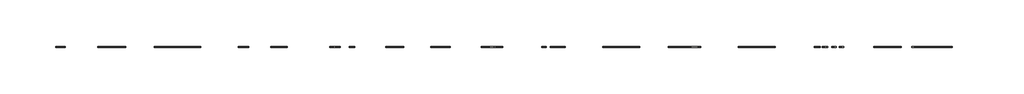
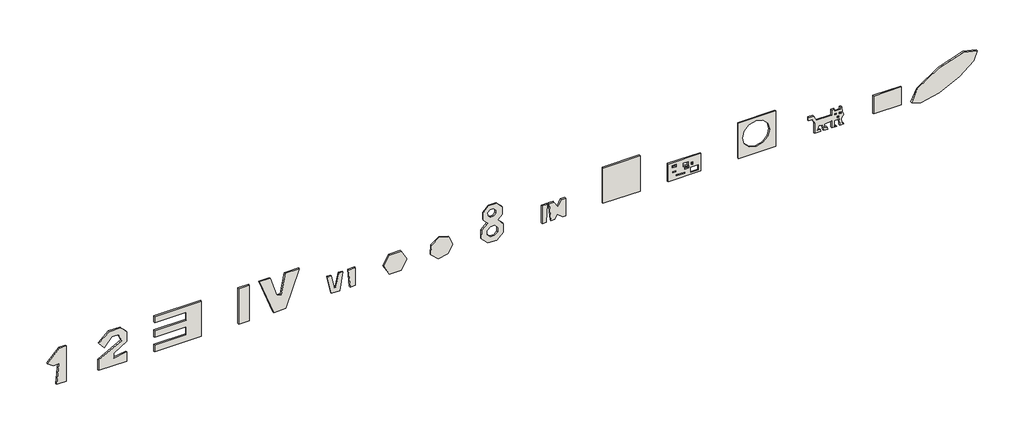
# One storey: 15 walls.
"""IFC4 building model written with IfcOpenShell, lengths in millimetres."""

from ifc_helpers import new_model, si_unit, point, frame, origin, origin_with_axes, place, context, project, spatial, polyline, ellipse_curve, trimmed, outline, extrude, element, save
from ifc_brep_helpers import plane_surface, extruded_surface, advanced_brep

model = new_model("IFC4")

# Units and contexts
model_context = context("Model", 3, world=origin())
ifc_project = project(units=[si_unit("LENGTHUNIT", "METRE", prefix="MILLI")], contexts=[model_context])

# Site, building, storey
site = spatial("IfcSite", under=ifc_project)
building = spatial("IfcBuilding", under=site)
storey = spatial("IfcBuildingStorey", under=building, Name="1 етаж", Elevation=0.0)

# Walls
placement = place(None, origin())
element("IfcWall", 1, ObjectType="Cav - 102 75i 100 p - Lwt", at=placement, inside=storey, context=model_context, shape_type="SweptSolid", body=[
    extrude(outline(polyline([(0.0, -98630.5096965), (8000.0, -98630.5096965), (8000.0, -100030.5096965), (5400.0, -102630.5096965), (4539.6353455, -101401.7816301), (4539.6353455, -100201.7816301), (0.0, -100630.5096965), (0.0, -98630.5096965)])), frame((0.0, 42970.9466245, 0.0), z_axis=(0.0, 1.0, 0.0), x_axis=(0.0, 0.0, 1.0)), (0.0, 0.0, 1.0), 290.0),
])
element("IfcWall", 2, ObjectType="Cav - 102 75i 100 p - Lwt", at=placement, inside=storey, context=model_context, shape_type="SweptSolid", body=[
    extrude(outline(polyline([(0.0, -91630.5096965), (0.0, -85630.5096965), (2094.5145842, -85630.5096965), (1651.266428, -88429.0684139), (2751.266428, -88429.0684139), (4500.0, -85630.5096965), (6700.0, -85630.5096965), (8000.0, -86930.5096965), (8000.0, -89366.1778706), (6130.4395076, -91594.233304), (4690.3678843, -90385.869736), (6660.3947683, -88846.7160477), (6660.3947683, -87446.7160477), (5029.0407516, -86686.0031765), (2400.0, -91630.5096965), (0.0, -91630.5096965)])), frame((0.0, 42970.9466245, 0.0), z_axis=(0.0, 1.0, 0.0), x_axis=(0.0, 0.0, 1.0)), (0.0, 0.0, 1.0), 290.0),
])
element("IfcWall", 3, ObjectType="Cav - 102 75i 100 p - Lwt", at=placement, inside=storey, context=model_context, shape_type="SweptSolid", body=[
    extrude(outline(polyline([(6600.0, -79630.5096965), (6600.0, -72830.5096965), (4800.0, -72830.5096965), (4800.0, -79630.5096965), (3300.0, -79630.5096965), (3300.0, -72830.5096965), (1500.0, -72830.5096965), (1500.0, -79630.5096965), (0.0, -79630.5096965), (0.0, -69630.5096965), (8000.0, -69630.5096965), (8000.0, -79630.5096965), (6600.0, -79630.5096965)])), frame((0.0, 42970.9466245, 0.0), z_axis=(0.0, 1.0, 0.0), x_axis=(0.0, 0.0, 1.0)), (0.0, 0.0, 1.0), 290.0),
])
element("IfcWall", 4, ObjectType="Cav - 102 75i 100 p - Lwt", at=placement, inside=storey, context=model_context, shape_type="SweptSolid", body=[
    extrude(outline(polyline([(-59330.5096965, 42970.9466245), (-61630.5096965, 42970.9466245), (-61630.5096965, 43260.9466245), (-59330.5096965, 43260.9466245), (-59330.5096965, 42970.9466245)])), origin_with_axes(), (0.0, 0.0, 1.0), 8000.0),
    extrude(outline(polyline([(8000.0, -51722.1990601), (3451.4918474, -52524.2237694), (3625.140025, -53509.0315224), (8000.0, -54930.5096965), (8000.0, -57230.5096965), (0.0, -54159.5974163), (0.0, -51542.2715707), (8000.0, -48630.5096965), (8000.0, -51722.1990601)])), frame((0.0, 42970.9466245, 0.0), z_axis=(0.0, 1.0, 0.0), x_axis=(0.0, 0.0, 1.0)), (0.0, 0.0, 1.0), 290.0),
])
element("IfcWall", 5, ObjectType="Cav - 102 75i 100 p - Lwt", at=placement, inside=storey, context=model_context, shape_type="SweptSolid", body=[
    extrude(outline(polyline([(4000.0, -36630.5096965), (4000.0, -38130.5096965), (0.0, -37780.5550424), (0.0, -36630.5096965), (4000.0, -36630.5096965)])), frame((0.0, 42970.9466245, 0.0), z_axis=(0.0, 1.0, 0.0), x_axis=(0.0, 0.0, 1.0)), (0.0, 0.0, 1.0), 290.0),
    extrude(outline(polyline([(0.0, -39964.0474578), (4000.0, -39330.5096965), (4000.0, -40183.0395516), (1065.5571978, -40806.7746241), (1065.5571978, -41206.7746241), (4000.0, -41830.5096965), (4000.0, -42630.5096965), (0.0, -41780.2834499), (0.0, -39964.0474578)])), frame((0.0, 42970.9466245, 0.0), z_axis=(0.0, 1.0, 0.0), x_axis=(0.0, 0.0, 1.0)), (0.0, 0.0, 1.0), 290.0),
])
element("IfcWall", 6, ObjectType="Cav - 102 75i 100 p - Lwt", at=placement, inside=storey, context=model_context, shape_type="SweptSolid", body=[
    extrude(outline(polyline([(21.877764, -26870.6721957), (2169.9022222, -25630.5096965), (4317.9266805, -26870.6721957), (4317.9266805, -29350.9971941), (2169.9022222, -30591.1596933), (21.877764, -29350.9971941), (21.877764, -26870.6721957)])), frame((0.0, 42970.9466245, 0.0), z_axis=(0.0, 1.0, 0.0), x_axis=(0.0, 0.0, 1.0)), (0.0, 0.0, 1.0), 290.0),
])
element("IfcWall", 7, ObjectType="Cav - 102 75i 100 p - Lwt", at=placement, inside=storey, context=model_context, shape_type="SweptSolid", body=[
    extrude(outline(polyline([(2063.3424206, -15809.1102472), (4000.0, -16630.5096965), (4565.2903012, -18656.7837428), (3333.5381977, -20362.1067006), (1232.2781465, -20462.3356006), (-156.1981759, -18881.9960367), (213.660221, -16811.1159336), (2063.3424206, -15809.1102472)])), frame((0.0, 42970.9466245, 0.0), z_axis=(0.0, 1.0, 0.0), x_axis=(0.0, 0.0, 1.0)), (0.0, 0.0, 1.0), 290.0),
])
element("IfcWall", 8, ObjectType="Cav - 102 75i 100 p - Lwt", at=placement, inside=storey, context=model_context, shape_type="SweptSolid", body=[
    extrude(outline(polyline([(6805.7289018, -5192.4839493), (8000.0, -6366.0908889), (8014.6117667, -8040.4335066), (6841.004827, -9234.7046048), (5166.6622094, -9249.3163715), (4214.4462038, -8313.576309), (3005.9972917, -9587.015755), (1085.0591362, -9637.3172909), (-308.8178169, -8314.5774521), (-359.1193527, -6393.6392966), (963.6204861, -4999.7623435), (2884.5586416, -4949.4608076), (4178.1921217, -6177.0731426), (5131.3862841, -5207.0957159), (6805.7289018, -5192.4839493)]), holes=[polyline([(5866.8485377, -6578.1456906), (5358.9896583, -7043.5126137), (5328.943308, -7731.6871783), (5794.3102311, -8239.5460576), (6482.4847957, -8269.592408), (6990.343675, -7804.2254848), (7020.3900254, -7116.0509203), (6555.0231022, -6608.1920409), (5866.8485377, -6578.1456906)]), polyline([(3115.8715667, -6771.7493574), (2438.7263942, -6151.2601266), (1521.1603081, -6191.321927), (900.6710773, -6868.4670995), (940.7328778, -7786.0331856), (1617.8780502, -8406.5224164), (2535.4441363, -8366.4606159), (3155.9333672, -7689.3154435), (3115.8715667, -6771.7493574)])]), frame((0.0, 42970.9466245, 0.0), z_axis=(0.0, 1.0, 0.0), x_axis=(0.0, 0.0, 1.0)), (0.0, 0.0, 1.0), 290.0),
])
element("IfcWall", 9, ObjectType="Cav - 102 75i 100 p - Lwt", at=placement, inside=storey, context=model_context, shape_type="SweptSolid", body=[
    extrude(outline(polyline([(0.0, 3369.4903035), (0.0, 4259.8591863), (4000.0, 4469.4903035), (4000.0, 3369.4903035), (0.0, 3369.4903035)])), frame((0.0, 42970.9466245, 0.0), z_axis=(0.0, 1.0, 0.0), x_axis=(0.0, 0.0, 1.0)), (0.0, 0.0, 1.0), 290.0),
    extrude(outline(polyline([(4000.0, 8369.4903035), (4000.0, 7408.7244661), (2643.1230461, 6717.3611262), (4000.0, 5869.4903035), (4000.0, 4869.4903035), (0.0, 5219.4449576), (0.0, 6089.0365293), (989.5288889, 6593.2266812), (0.0, 7772.5012895), (0.0, 8369.4903035), (4000.0, 8369.4903035)])), frame((0.0, 42970.9466245, 0.0), z_axis=(0.0, 1.0, 0.0), x_axis=(0.0, 0.0, 1.0)), (0.0, 0.0, 1.0), 290.0),
])
element("IfcWall", 10, ObjectType="Cav - 102 75i 100 p - Lwt", at=placement, inside=storey, context=model_context, shape_type="SweptSolid", body=[
    extrude(outline(polyline([(24369.4903035, 42970.9466245), (16369.4903035, 42970.9466245), (16369.4903035, 43260.9466245), (24369.4903035, 43260.9466245), (24369.4903035, 42970.9466245)])), origin_with_axes(), (0.0, 0.0, 1.0), 8000.0),
])
element("IfcWall", 11, ObjectType="Cav - 102 75i 100 p - Lwt", at=placement, inside=storey, context=model_context, shape_type="SweptSolid", body=[
    extrude(outline(polyline([(0.0, 30369.4903035), (0.0, 37369.4903035), (4000.0, 37369.4903035), (4000.0, 30369.4903035), (0.0, 30369.4903035)]), holes=[polyline([(3368.16, 32060.8162862), (2868.16, 32060.8162862), (2868.16, 31260.8162862), (3368.16, 31260.8162862), (3368.16, 32060.8162862)]), polyline([(3099.8933333, 34632.1407307), (2299.8933333, 34632.1407307), (2299.8933333, 33532.1407307), (3099.8933333, 33532.1407307), (3099.8933333, 34632.1407307)]), polyline([(962.7022222, 33860.8162862), (762.7022222, 33860.8162862), (762.7022222, 32060.8162862), (962.7022222, 32060.8162862), (962.7022222, 33860.8162862)]), polyline([(1651.2533333, 36822.2207307), (451.2533333, 36822.2207307), (451.2533333, 35222.2207307), (1651.2533333, 35222.2207307), (1651.2533333, 36822.2207307)]), polyline([(2688.5511111, 35324.6207307), (2688.5511111, 35624.6207307), (2188.5511111, 35624.6207307), (2188.5511111, 35324.6207307), (2688.5511111, 35324.6207307)]), polyline([(2125.1911111, 33860.8162862), (2125.1911111, 34703.5718418), (1651.2533333, 34703.5718418), (1651.2533333, 33860.8162862), (2125.1911111, 33860.8162862)]), polyline([(1731.7333333, 31331.4829529), (1931.7333333, 31331.4829529), (1931.7333333, 31931.4829529), (1731.7333333, 31931.4829529), (1731.7333333, 31331.4829529)])]), frame((0.0, 42970.9466245, 0.0), z_axis=(0.0, 1.0, 0.0), x_axis=(0.0, 0.0, 1.0)), (0.0, 0.0, 1.0), 290.0),
])
element("IfcWall", 12, ObjectType="Cav - 102 75i 100 p - Lwt", at=placement, inside=storey, context=model_context, shape_type="SweptSolid", body=[
    extrude(outline(polyline([(0.0, 45369.4903035), (0.0, 53369.4903035), (8000.0, 53369.4903035), (8000.0, 45369.4903035), (0.0, 45369.4903035)]), holes=[polyline([(4318.9511111, 52086.5671726), (2869.5644585, 51698.2051895), (1808.539789, 50637.18052), (1420.177806, 49187.7938674), (1808.539789, 47738.4072148), (2869.5644585, 46677.3825453), (4318.9511111, 46289.0205623), (5768.3377637, 46677.3825453), (6829.3624332, 47738.4072148), (7217.7244163, 49187.7938674), (6829.3624332, 50637.18052), (5768.3377637, 51698.2051895), (4318.9511111, 52086.5671726)])]), frame((0.0, 42970.9466245, 0.0), z_axis=(0.0, 1.0, 0.0), x_axis=(0.0, 0.0, 1.0)), (0.0, 0.0, 1.0), 290.0),
])
element("IfcWall", 13, ObjectType="Cav - 102 75i 100 p - Lwt", at=placement, inside=storey, context=model_context, shape_type="SweptSolid", body=[
    extrude(outline(polyline([(3300.0, 60369.4903035), (3300.0, 61169.4903035), (2337.9183221, 61702.7808857), (0.0, 61702.7808857), (0.0, 62998.7101733), (482.9629131, 62869.3006507), (535.2563588, 62271.5838319), (1458.9577164, 62607.7836314), (1337.403992, 63297.1490585), (0.0, 63655.5053781), (0.0, 64502.7808857), (482.9629131, 64373.3713632), (688.1749991, 63809.5557907), (1385.5112878, 63748.5467708), (1527.3254711, 65369.4903035), (0.0, 65369.4903035), (0.0, 66420.201364), (318.1483442, 65869.1522675), (1418.1483442, 65869.1522675), (1418.1483442, 66969.1522675), (0.0, 67093.2241708), (0.0, 67969.4903035), (494.9747468, 67474.5155566), (1418.1483442, 67393.7483324), (2155.3851841, 67909.9671251), (2816.8665248, 67587.3411185), (4000.0, 67483.830352), (4000.0, 67169.4903035), (3500.0, 67169.4903035), (3500.0, 65969.4903035), (4000.0, 65969.4903035), (4000.0, 65369.4903035), (2800.0, 65369.4903035), (2800.0, 62069.4903035), (4000.0, 61484.2111972), (4000.0, 60369.4903035), (3300.0, 60369.4903035)]), holes=[polyline([(2950.3577045, 66363.1028194), (2650.3577045, 66363.1028194), (2650.3577045, 66063.1028194), (2950.3577045, 66063.1028194), (2950.3577045, 66363.1028194)]), polyline([(2950.3577045, 67384.3679411), (2550.3577045, 67384.3679411), (2550.3577045, 66984.3679411), (2950.3577045, 66984.3679411), (2950.3577045, 67384.3679411)]), polyline([(2164.8579691, 66909.1890889), (1864.8579691, 66909.1890889), (1864.8579691, 66509.1890889), (2164.8579691, 66509.1890889), (2164.8579691, 66909.1890889)])]), frame((0.0, 42970.9466245, 0.0), z_axis=(0.0, 1.0, 0.0), x_axis=(0.0, 0.0, 1.0)), (0.0, 0.0, 1.0), 290.0),
])
element("IfcWall", 14, ObjectType="Cav - 102 75i 100 p - Lwt", at=placement, inside=storey, context=model_context, shape_type="SweptSolid", body=[
    extrude(outline(polyline([(80296.0426464, 42970.9466245), (74369.4903035, 42970.9466245), (74369.4903035, 43260.9466245), (80296.0426464, 43260.9466245), (80296.0426464, 42970.9466245)])), origin_with_axes(), (0.0, 0.0, 1.0), 4000.0),
])
element("IfcWall", 15, ObjectType="Cav - 102 75i 100 p - Lwt", at=placement, inside=storey, context=model_context, shape_type="AdvancedBrep", body=[
    advanced_brep(
    [(96500.2659618, 42970.9466245, 6549.4282783), (82479.0788395, 42970.9466245, -289.1616116), (96500.2659618, 43260.9466245, 6549.4282783), (82479.0788395, 43260.9466245, -289.1616116)],
    [
        (0, 1, ellipse_curve(frame((89489.6724007, 42970.9466245, 3130.1333333), z_axis=(0.0, -1.0000000000000002, 0.0), x_axis=(-0.8987940462991659, 0.0, -0.4383711467890798)), 7800.0, 2600.0)),
        (1, 0, ellipse_curve(frame((89489.6724007, 42970.9466245, 3130.1333333), z_axis=(0.0, -1.0000000000000002, 0.0), x_axis=(-0.8987940462991659, 0.0, -0.4383711467890798)), 7800.0, 2600.0)),
        (2, 3, ellipse_curve(frame((89489.6724007, 43260.9466245, 3130.1333333), z_axis=(0.0, 1.0000000000000002, 0.0), x_axis=(-0.8987940462991659, 0.0, -0.4383711467890798)), 7800.0, 2600.0)),
        (3, 2, ellipse_curve(frame((89489.6724007, 43260.9466245, 3130.1333333), z_axis=(0.0, 1.0000000000000002, 0.0), x_axis=(-0.8987940462991659, 0.0, -0.4383711467890798)), 7800.0, 2600.0)),
        (0, 2),
        (3, 1),
    ],
    [
        plane_surface(frame((82479.0788395, 42970.9466245, -289.1616116), z_axis=(0.0, -1.0000000000000002, 0.0), x_axis=(0.4383711467890798, 0.0, -0.8987940462991659))),
        plane_surface(frame((82479.0788395, 43260.9466245, -289.1616116), z_axis=(0.0, 1.0000000000000002, 0.0), x_axis=(-0.4383711467890798, 0.0, 0.8987940462991659))),
        extruded_surface(trimmed(ellipse_curve(frame((89489.6724007, 43550.9466245, 3130.1333333), z_axis=(0.0, -1.0000000000000002, 0.0), x_axis=(-0.8987940462991659, 0.0, -0.4383711467890798)), 7800.0, 2600.0), [point((96500.2659618, 43550.9466245, 6549.4282783))], [point((82479.0788395, 43550.9466245, -289.1616116))], True, "CARTESIAN"), (0.0, -290.0, 0.0), 290.0),
        extruded_surface(trimmed(ellipse_curve(frame((89489.6724007, 43550.9466245, 3130.1333333), z_axis=(0.0, -1.0000000000000002, 0.0), x_axis=(-0.8987940462991659, 0.0, -0.4383711467890798)), 7800.0, 2600.0), [point((82479.0788395, 43550.9466245, -289.1616116))], [point((96500.2659618, 43550.9466245, 6549.4282783))], True, "CARTESIAN"), (0.0, -290.0, 0.0), 290.0),
    ],
    [
        (0, [[1, 2]]),
        (1, [[3, 4]]),
        (2, [[-1, 5, -4, 6]]),
        (3, [[-2, -6, -3, -5]]),
    ],
),
])

save(model, "model.ifc")

# Revit data of these elements
# Project information
#   Project Issue Date = "Issue Date"
#   Project Status = "Project Status"
#   Client Name = "Owner"
#   Project Address = "Enter address here"
#   Project Name = "Project Name"
#   Project Number = "Project Number"
# Type "Cav - 102 75i 100 p - Lwt"
#   Keynote = "F10"
#   Layers, outside or top first: 10.25 cm "Masonry - Brick" (function 4); 7.5 cm "Insulation / Thermal Barriers - Batt insulation" (function 3); 10 cm "Masonry - Concrete Block" (function 1); 1.25 cm "Plasterboard" (function 5)
# Elements 1, 2, 3, 4, 8, 10, 12, 15 (IfcWall, "Cav - 102 75i 100 p - Lwt")
#   Top Offset = 0 cm
#   Base Offset = 0 cm
#   Unconnected Height = 800 cm
#   wall height = 800 cm
#   Phase Created = New Construction
#   Base Constraint = 1 етаж
#   Materials on its faces: "Default Wall", "Masonry - Brick", "Plasterboard"
# Elements 5, 6, 7, 9, 11, 13, 14 (IfcWall, "Cav - 102 75i 100 p - Lwt")
#   Top Offset = 0 cm
#   Base Offset = 0 cm
#   Unconnected Height = 400 cm
#   wall height = 400 cm
#   Phase Created = New Construction
#   Base Constraint = 1 етаж
#   Materials on its faces: "Default Wall", "Masonry - Brick", "Plasterboard"
# Materials
#   "Masonry - Brick": class "Brick", colour RGB 170 100 105, transparency 0, Keynote = "F10", Cost = 0
#   "Insulation / Thermal Barriers - Batt insulation": class "Miscellaneous", colour RGB 127 127 127, transparency 0, Keynote = "P11", Comments = "Rendering appearance not upgraded "
#   "Masonry - Concrete Block": class "Concrete", colour RGB 181 181 181, transparency 0, Keynote = "F10"
#   "Plasterboard": class "Drywall", colour RGB 249 249 249, transparency 0, Keynote = "K10", Description = "Interior finish"
#   "Default Wall": class "Miscellaneous", colour RGB 128 128 128, transparency 0, Comments = "Rendering appearance not upgraded "
